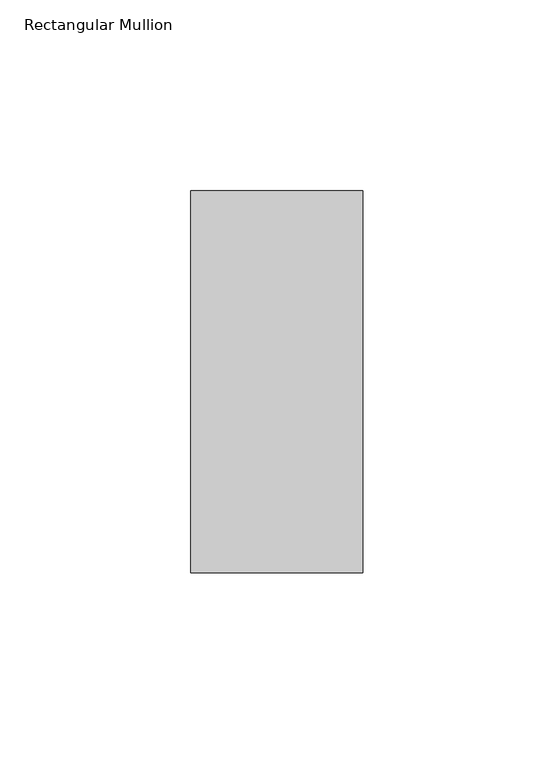
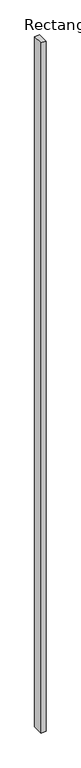
"""IFC4 building model written with IfcOpenShell, lengths in millimetres: member geometry, Rectangular Mullion : 알루미늄_Rectangular Cap_100 x 45."""

from ifc_helpers import new_model, si_unit, frame, origin, place, context, project, spatial, polyline, outline, extrude, source, transform, mapped, element, save


def rectangular_mullion_d4d12df6(model_context):
    return source(origin(), model_context, "Body", "SweptSolid", [
        extrude(outline(polyline([(0.0, 50.0), (0.0, -50.0), (-45.0, -50.0), (-45.0, 50.0), (0.0, 50.0)])), frame((0.0, 0.0, -6569.0), z_axis=(0.0, 0.0, 1.0), x_axis=(1.0, 0.0, 0.0)), (0.0, 0.0, 1.0), 6569.0),
    ])


if __name__ == "__main__":
    model = new_model("IFC4")
    model_context = context("Model", 3, world=origin())
    ifc_project = project(units=[si_unit("LENGTHUNIT", "METRE", prefix="MILLI")], contexts=[model_context])
    site = spatial("IfcSite", under=ifc_project)
    building = spatial("IfcBuilding", under=site)
    placement = place(None, origin())
    rectangular_mullion_shape = rectangular_mullion_d4d12df6(model_context)
    element("IfcMember", 1, ObjectType="Rectangular Mullion : 알루미늄_Rectangular Cap_100 x 45", at=placement, inside=building, context=model_context, shape_type="MappedRepresentation", body=[
        mapped(rectangular_mullion_shape, transform((0.0, 0.0, 0.0), x_axis=(1.0, 0.0, 0.0), y_axis=(0.0, 1.0, 0.0), z_axis=(0.0, 0.0, 1.0))),
    ])
    save(model, "model.ifc")

# Revit data of these elements
# Type "Rectangular Mullion : 알루미늄_Rectangular Cap_100 x 45"
#   built-in parameter 1007304 = 0.328084 (stored number, unit not read)
#   built-in parameter 1007301 = 0.0738189 (stored number, unit not read)
#   built-in parameter 1007300 = 0.0738189 (stored number, unit not read)
# Element 1 (IfcMember, "Rectangular Mullion : 알루미늄_Rectangular Cap_100 x 45")
#   Materials on its faces: "00_Metal_Stainless Steel"
# Materials
#   "00_Metal_Stainless Steel": class "Metal", colour RGB 148 148 148, transparency 0, Description = "Steel", Cost = 0
